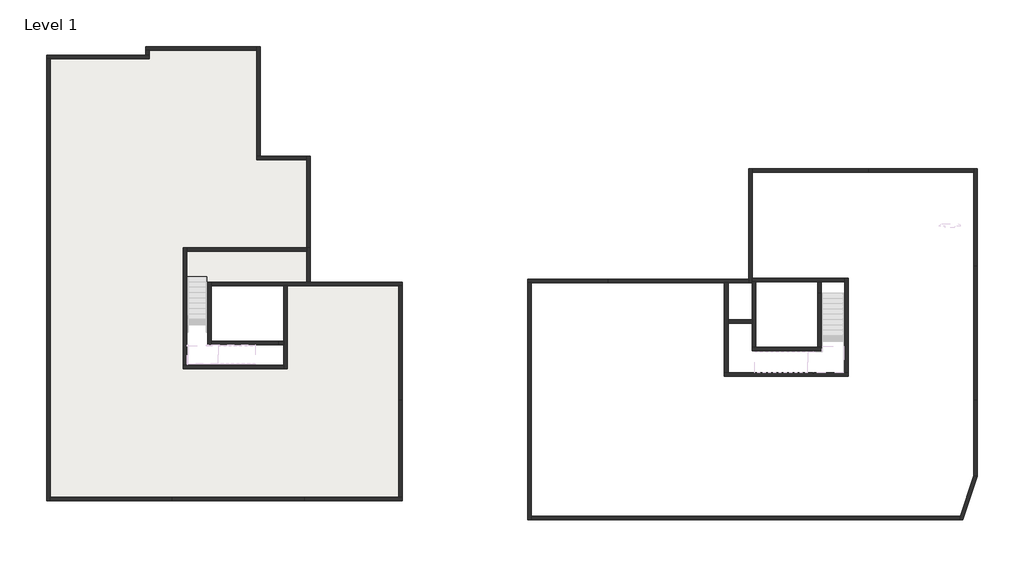
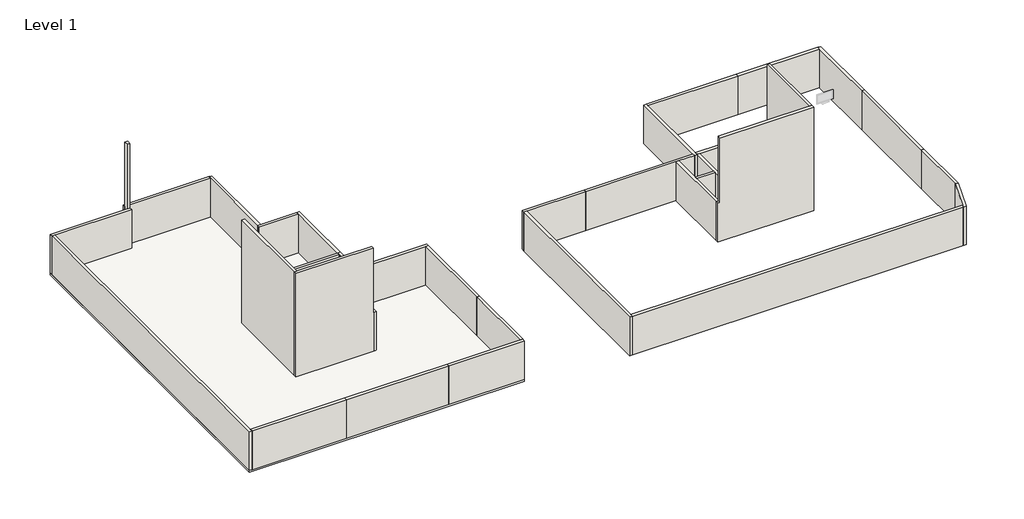
# One storey, part 1 of 2: 41 walls, 1 slab.
"""IFC4 building model written with IfcOpenShell, lengths in millimetres."""

from ifc_helpers import new_model, si_unit, frame, origin, origin_with_axes, place, context, project, spatial, polyline, outline, extrude, faceted_brep, element, save

model = new_model("IFC4")

# Units and contexts
model_context = context("Model", 3, world=origin())
ifc_project = project(units=[si_unit("LENGTHUNIT", "METRE", prefix="MILLI")], contexts=[model_context])

# Site, building, storey
site = spatial("IfcSite", under=ifc_project)
building = spatial("IfcBuilding", under=site)
storey = spatial("IfcBuildingStorey", under=building, Name="Level 1", Elevation=0.0)

# Slab
placement = place(None, origin())
element("IfcSlab", 1, ObjectType="Generic 150mm", at=placement, inside=storey, context=model_context, shape_type="SweptSolid", body=[
    extrude(outline(polyline([(-16680.1759629, 14256.1136739), (-16680.1759629, 14747.088776), (-10220.690523, 14747.088776), (-10220.690523, 8542.3434304), (-7387.4411293, 8542.3434304), (-7387.4411293, 1427.088776), (-2180.690523, 1427.088776), (-2180.690523, -10932.392509), (-22296.8569344, -10932.392509), (-22296.8569344, 14256.1136739), (-16680.1759629, 14256.1136739)]), holes=[polyline([(-8880.690523, -3253.8863261), (-8880.690523, 1227.088776), (-8880.690523, 1427.088776), (-14380.690523, 1427.088776), (-14380.690523, -3253.8863261), (-8880.690523, -3253.8863261)])]), frame((0.0, 0.0, -150.0), z_axis=(0.0, 0.0, 1.0), x_axis=(1.0, 0.0, 0.0)), (0.0, 0.0, 1.0), 150.0),
])

# Walls
element("IfcWall", 2, ObjectType="Generic - 200mm", at=placement, inside=storey, context=model_context, shape_type="SweptSolid", body=[
    extrude(outline(polyline([(30117.9969803, 7645.7271169), (24149.836337, 7645.7271169), (24149.836337, 7845.7271169), (30117.9969803, 7845.7271169), (30117.9969803, 7645.7271169)])), origin_with_axes(), (0.0, 0.0, 1.0), 3000.0),
])
element("IfcWall", 3, ObjectType="Generic - 200mm", at=placement, inside=storey, context=model_context, shape_type="Brep", body=[
    faceted_brep([(30117.9969803, 7845.7271169, 0.0), (30117.9969803, 7645.7271169, 0.0), (30117.9969803, 2319.475628, 0.0), (30117.9969803, 2319.475628, 3000.0), (30117.9969803, 7645.7271169, 3000.0), (30117.9969803, 7845.7271169, 3000.0), (30317.9969803, 7845.7271169, 0.0), (30317.9969803, 7845.7271169, 3000.0), (30317.9969803, 2319.475628, 3000.0), (30317.9969803, 2319.475628, 0.0), (30118.5156953, 2319.475628, 0.0), (30268.3425199, 2319.475628, 3000.0), (30118.5156953, 2319.475628, 3000.0)], [[[0, 1, 2, 3, 4, 5]], [[6, 7, 8, 9]], [[2, 1, 0, 6, 9, 10]], [[3, 2, 10, 9, 8, 11, 12]], [[5, 4, 3, 12, 11, 8, 7]], [[0, 5, 7, 6]]]),
])
element("IfcWall", 4, ObjectType="Generic - 200mm", at=placement, inside=storey, context=model_context, shape_type="Brep", body=[
    faceted_brep([(30118.5156953, 2319.475628, 0.0), (30118.5156953, -5240.0098119, 0.0), (30118.5156953, -5240.0098119, 3000.0), (30118.5156953, 2319.475628, 3000.0), (30318.5156953, 2319.475628, 0.0), (30318.5156953, 2319.475628, 3000.0), (30318.5156953, -5240.0098119, 3000.0), (30318.5156953, -5240.0098119, 0.0), (30317.9969803, 2319.475628, 0.0), (30119.0344102, -5240.0098119, 0.0), (30268.8612349, -5240.0098119, 3000.0), (30119.0344102, -5240.0098119, 3000.0), (30317.9969803, 2319.475628, 3000.0), (30268.8612349, 2319.475628, 3000.0)], [[[0, 1, 2, 3]], [[4, 5, 6, 7]], [[1, 0, 8, 4, 7, 9]], [[2, 1, 9, 7, 6, 10, 11]], [[3, 2, 11, 10, 6, 5, 12, 13]], [[0, 3, 13, 12, 5, 4, 8]]]),
])
element("IfcWall", 5, ObjectType="Generic - 200mm", at=placement, inside=storey, context=model_context, shape_type="Brep", body=[
    faceted_brep([(30119.0344102, -5240.0098119, 0.0), (30119.0344102, -9516.773704, 0.0), (30119.0344102, -9516.773704, 3000.0), (30119.0344102, -5240.0098119, 3000.0), (30319.0344102, -5240.0098119, 0.0), (30319.0344102, -5240.0098119, 3000.0), (30319.0344102, -9549.611954, 3000.0), (30319.0344102, -9549.611954, 0.0), (30318.5156953, -5240.0098119, 0.0), (30318.5156953, -5240.0098119, 3000.0), (30269.3799498, -5240.0098119, 3000.0)], [[[0, 1, 2, 3]], [[4, 5, 6, 7]], [[1, 0, 8, 4, 7]], [[3, 2, 6, 5, 9, 10]], [[0, 3, 10, 9, 5, 4, 8]], [[2, 1, 7, 6]]]),
])
element("IfcWall", 6, ObjectType="Generic - 200mm", at=placement, inside=storey, context=model_context, shape_type="Brep", body=[
    faceted_brep([(21499.4907974, -2250.0293367, 0.0), (21299.4907974, -2250.0293367, 0.0), (17780.2585618, -2250.0293367, 0.0), (17580.2585618, -2250.0293367, 0.0), (17580.2585618, -2250.0293367, 3000.0), (17780.2585618, -2250.0293367, 3000.0), (21299.4907974, -2250.0293367, 3000.0), (21499.4907974, -2250.0293367, 3000.0), (21499.4907974, -2450.0293367, 0.0), (21499.4907974, -2450.0293367, 3000.0), (17580.2585618, -2450.0293367, 3000.0), (17580.2585618, -2450.0293367, 0.0)], [[[0, 1, 2, 3, 4, 5, 6, 7]], [[8, 9, 10, 11]], [[3, 2, 1, 0, 8, 11]], [[7, 6, 5, 4, 10, 9]], [[4, 3, 11, 10]], [[0, 7, 9, 8]]]),
])
element("IfcWall", 7, ObjectType="Generic - 200mm", at=placement, inside=storey, context=model_context, shape_type="SweptSolid", body=[
    extrude(outline(polyline([(5093.3704674, -11810.4392945), (29344.9668625, -11810.4392945), (29277.4707506, -12010.4392945), (5093.3704674, -12010.4392945), (5093.3704674, -11810.4392945)])), origin_with_axes(), (0.0, 0.0, 1.0), 3000.0),
])
element("IfcWall", 8, ObjectType="Generic - 200mm", at=placement, inside=storey, context=model_context, shape_type="Brep", body=[
    faceted_brep([(30119.0344102, -9516.773704, 0.0), (29344.9668625, -11810.4392945, 0.0), (29277.4707506, -12010.4392945, 0.0), (29277.4707506, -12010.4392945, 3000.0), (29344.9668625, -11810.4392945, 3000.0), (30119.0344102, -9516.773704, 3000.0), (30319.0344102, -9549.611954, 0.0), (30319.0344102, -9549.611954, 3000.0), (29488.5530216, -12010.4392945, 3000.0), (29488.5530216, -12010.4392945, 0.0)], [[[0, 1, 2, 3, 4, 5]], [[6, 7, 8, 9]], [[2, 1, 0, 6, 9]], [[5, 4, 3, 8, 7]], [[0, 5, 7, 6]], [[3, 2, 9, 8]]]),
])
element("IfcWall", 9, ObjectType="Generic - 200mm", at=placement, inside=storey, context=model_context, shape_type="Brep", body=[
    faceted_brep([(4893.3704674, 1406.241677, 0.0), (4893.3704674, -12010.4392945, 0.0), (4893.3704674, -12010.4392945, 3000.0), (4893.3704674, 1406.241677, 3000.0), (5093.3704674, 1406.241677, 0.0), (5093.3704674, 1406.241677, 3000.0), (5093.3704674, -11810.4392945, 3000.0), (5093.3704674, -12010.4392945, 3000.0), (5093.3704674, -12010.4392945, 0.0), (5093.3704674, -11810.4392945, 0.0)], [[[0, 1, 2, 3]], [[4, 5, 6, 7, 8, 9]], [[1, 0, 4, 9, 8]], [[3, 2, 7, 6, 5]], [[2, 1, 8, 7]], [[0, 3, 5, 4]]]),
])
element("IfcWall", 10, ObjectType="Generic - 200mm", at=placement, inside=storey, context=model_context, shape_type="Brep", body=[
    faceted_brep([(21299.4907974, 799.475628, 0.0), (21299.4907974, -2250.0293367, 0.0), (21299.4907974, -2250.0293367, 3000.0), (21299.4907974, 799.475628, 3000.0), (21499.4907974, 799.475628, 0.0), (21499.4907974, 799.475628, 3000.0), (21499.4907974, -2250.0293367, 3000.0), (21499.4907974, -2250.0293367, 0.0), (21449.836337, 799.475628, 3000.0)], [[[0, 1, 2, 3]], [[4, 5, 6, 7]], [[1, 0, 4, 7]], [[3, 2, 6, 5, 8]], [[0, 3, 8, 5, 4]], [[2, 1, 7, 6]]]),
])
element("IfcWall", 11, ObjectType="Generic - 200mm", at=placement, inside=storey, context=model_context, shape_type="Brep", body=[
    faceted_brep([(17580.2585618, 1445.7271169, 0.0), (17580.2585618, -694.2728831, 0.0), (17580.2585618, -894.2728831, 0.0), (17580.2585618, -2250.0293367, 0.0), (17580.2585618, -2250.0293367, 3000.0), (17580.2585618, -894.2728831, 3000.0), (17580.2585618, -694.2728831, 3000.0), (17580.2585618, 1445.7271169, 3000.0), (17780.2585618, 1445.7271169, 0.0), (17780.2585618, 1445.7271169, 3000.0), (17780.2585618, -2250.0293367, 3000.0), (17780.2585618, -2250.0293367, 0.0)], [[[0, 1, 2, 3, 4, 5, 6, 7]], [[8, 9, 10, 11]], [[3, 2, 1, 0, 8, 11]], [[7, 6, 5, 4, 10, 9]], [[0, 7, 9, 8]], [[4, 3, 11, 10]]]),
])
element("IfcWall", 12, ObjectType="Generic - 200mm", at=placement, inside=storey, context=model_context, shape_type="Brep", body=[
    faceted_brep([(21499.4907974, 799.475628, 0.0), (21499.4907974, 1445.7271169, 0.0), (21499.4907974, 1445.7271169, 3000.0), (21499.4907974, 799.475628, 3000.0), (21299.4907974, 799.475628, 0.0), (21299.4907974, 799.475628, 3000.0), (21299.4907974, 1445.7271169, 3000.0), (21299.4907974, 1445.7271169, 0.0), (21449.836337, 799.475628, 3000.0)], [[[0, 1, 2, 3]], [[4, 5, 6, 7]], [[1, 0, 4, 7]], [[3, 2, 6, 5, 8]], [[0, 3, 8, 5, 4]], [[2, 1, 7, 6]]]),
])
element("IfcWall", 13, ObjectType="Generic - 200mm", at=placement, inside=storey, context=model_context, shape_type="SweptSolid", body=[
    extrude(outline(polyline([(24149.836337, 7645.7271169), (17578.5156953, 7645.7271169), (17578.5156953, 7845.7271169), (24149.836337, 7845.7271169), (24149.836337, 7645.7271169)])), origin_with_axes(), (0.0, 0.0, 1.0), 3000.0),
])
element("IfcWall", 14, ObjectType="Generic - 200mm", at=placement, inside=storey, context=model_context, shape_type="Brep", body=[
    faceted_brep([(16220.2585618, -3694.2728831, 0.0), (16220.2585618, -894.2728831, 0.0), (16220.2585618, -694.2728831, 0.0), (16220.2585618, 1405.7271169, 0.0), (16220.2585618, 1405.7271169, 3000.0), (16220.2585618, -694.2728831, 3000.0), (16220.2585618, -894.2728831, 3000.0), (16220.2585618, -3694.2728831, 3000.0), (16020.2585618, -3694.2728831, 0.0), (16020.2585618, -3694.2728831, 3000.0), (16020.2585618, 1405.7271169, 3000.0), (16020.2585618, 1405.7271169, 0.0), (16170.6041014, -3694.2728831, 3000.0)], [[[0, 1, 2, 3, 4, 5, 6, 7]], [[8, 9, 10, 11]], [[3, 2, 1, 0, 8, 11]], [[7, 6, 5, 4, 10, 9, 12]], [[4, 3, 11, 10]], [[0, 7, 12, 9, 8]]]),
])
element("IfcWall", 15, ObjectType="Generic - 200mm", at=placement, inside=storey, context=model_context, shape_type="SweptSolid", body=[
    extrude(outline(polyline([(17580.2585618, -894.2728831), (16220.2585618, -894.2728831), (16220.2585618, -694.2728831), (17580.2585618, -694.2728831), (17580.2585618, -894.2728831)])), origin_with_axes(), (0.0, 0.0, 1.0), 3000.0),
])
element("IfcWall", 16, ObjectType="Generic - 200mm", at=placement, inside=storey, context=model_context, shape_type="Brep", body=[
    faceted_brep([(17378.5156953, 7845.7271169, 0.0), (17378.5156953, 1605.7271169, 0.0), (17378.5156953, 1405.7271169, 0.0), (17378.5156953, 1405.7271169, 3000.0), (17378.5156953, 1605.7271169, 3000.0), (17378.5156953, 7845.7271169, 3000.0), (17578.5156953, 7845.7271169, 0.0), (17578.5156953, 7845.7271169, 3000.0), (17578.5156953, 7645.7271169, 3000.0), (17578.5156953, 1645.7271169, 3000.0), (17578.5156953, 1445.7271169, 3000.0), (17578.5156953, 1405.7271169, 3000.0), (17578.5156953, 1405.7271169, 0.0), (17578.5156953, 1445.7271169, 0.0), (17578.5156953, 1645.7271169, 0.0), (17578.5156953, 7645.7271169, 0.0)], [[[0, 1, 2, 3, 4, 5]], [[6, 7, 8, 9, 10, 11, 12, 13, 14, 15]], [[2, 1, 0, 6, 15, 14, 13, 12]], [[5, 4, 3, 11, 10, 9, 8, 7]], [[0, 5, 7, 6]], [[3, 2, 12, 11]]]),
])
element("IfcWall", 17, ObjectType="Generic - 200mm", at=placement, inside=storey, context=model_context, shape_type="Brep", body=[
    faceted_brep([(17378.5156953, 1605.7271169, 0.0), (9418.5156953, 1605.7271169, 0.0), (9418.5156953, 1605.7271169, 3000.0), (17378.5156953, 1605.7271169, 3000.0), (17378.5156953, 1405.7271169, 0.0), (17378.5156953, 1405.7271169, 3000.0), (16220.2585618, 1405.7271169, 3000.0), (16020.2585618, 1405.7271169, 3000.0), (9418.5156953, 1405.7271169, 3000.0), (9418.5156953, 1405.7271169, 0.0), (16020.2585618, 1405.7271169, 0.0), (16220.2585618, 1405.7271169, 0.0), (9418.5156953, 1406.241677, 0.0), (9418.5156953, 1406.241677, 3000.0)], [[[0, 1, 2, 3]], [[4, 5, 6, 7, 8, 9, 10, 11]], [[1, 0, 4, 11, 10, 9, 12]], [[2, 1, 12, 9, 8, 13]], [[3, 2, 13, 8, 7, 6, 5]], [[0, 3, 5, 4]]]),
])
element("IfcWall", 18, ObjectType="Generic - 200mm", at=placement, inside=storey, context=model_context, shape_type="Brep", body=[
    faceted_brep([(22820.2585618, 1645.7271169, 0.0), (17578.5156953, 1645.7271169, 0.0), (17578.5156953, 1645.7271169, 3000.0), (22820.2585618, 1645.7271169, 3000.0), (22820.2585618, 1445.7271169, 0.0), (22820.2585618, 1445.7271169, 3000.0), (21499.4907974, 1445.7271169, 3000.0), (21299.4907974, 1445.7271169, 3000.0), (17780.2585618, 1445.7271169, 3000.0), (17580.2585618, 1445.7271169, 3000.0), (17578.5156953, 1445.7271169, 3000.0), (17578.5156953, 1445.7271169, 0.0), (17580.2585618, 1445.7271169, 0.0), (17780.2585618, 1445.7271169, 0.0), (21299.4907974, 1445.7271169, 0.0), (21499.4907974, 1445.7271169, 0.0)], [[[0, 1, 2, 3]], [[4, 5, 6, 7, 8, 9, 10, 11, 12, 13, 14, 15]], [[1, 0, 4, 15, 14, 13, 12, 11]], [[3, 2, 10, 9, 8, 7, 6, 5]], [[2, 1, 11, 10]], [[0, 3, 5, 4]]]),
])
element("IfcWall", 19, ObjectType="Generic - 200mm", at=placement, inside=storey, context=model_context, shape_type="SweptSolid", body=[
    extrude(outline(polyline([(-2380.690523, -10732.392509), (-2380.690523, -5240.1378151), (-2180.690523, -5240.1378151), (-2180.690523, -10732.392509), (-2380.690523, -10732.392509)])), origin_with_axes(), (0.0, 0.0, 1.0), 3000.0),
])
element("IfcWall", 20, ObjectType="Generic - 200mm", at=placement, inside=storey, context=model_context, shape_type="Brep", body=[
    faceted_brep([(-2180.690523, -10732.392509, 0.0), (-2380.690523, -10732.392509, 0.0), (-7730.3449834, -10732.392509, 0.0), (-7730.3449834, -10732.392509, 3000.0), (-2380.690523, -10732.392509, 3000.0), (-2180.690523, -10732.392509, 3000.0), (-2180.690523, -10932.392509, 0.0), (-2180.690523, -10932.392509, 3000.0), (-7730.3449834, -10932.392509, 3000.0), (-7730.3449834, -10932.392509, 0.0), (-7730.3449834, -10732.911224, 0.0), (-7730.3449834, -10758.643998, 3000.0), (-7730.3449834, -10732.911224, 3000.0)], [[[0, 1, 2, 3, 4, 5]], [[6, 7, 8, 9]], [[2, 1, 0, 6, 9, 10]], [[3, 2, 10, 9, 8, 11, 12]], [[5, 4, 3, 12, 11, 8, 7]], [[0, 5, 7, 6]]]),
])
element("IfcWall", 21, ObjectType="Generic - 200mm", at=placement, inside=storey, context=model_context, shape_type="Brep", body=[
    faceted_brep([(-7730.3449834, -10732.911224, 0.0), (-15209.8304233, -10732.911224, 0.0), (-15209.8304233, -10732.911224, 3000.0), (-7730.3449834, -10732.911224, 3000.0), (-7730.3449834, -10932.911224, 0.0), (-7730.3449834, -10932.911224, 3000.0), (-15209.8304233, -10932.911224, 3000.0), (-15209.8304233, -10932.911224, 0.0), (-7730.3449834, -10932.392509, 0.0), (-15209.8304233, -10733.429939, 0.0), (-15209.8304233, -10759.1627129, 3000.0), (-15209.8304233, -10733.429939, 3000.0), (-7730.3449834, -10932.392509, 3000.0), (-7730.3449834, -10759.1627129, 3000.0)], [[[0, 1, 2, 3]], [[4, 5, 6, 7]], [[1, 0, 8, 4, 7, 9]], [[2, 1, 9, 7, 6, 10, 11]], [[3, 2, 11, 10, 6, 5, 12, 13]], [[0, 3, 13, 12, 5, 4, 8]]]),
])
element("IfcWall", 22, ObjectType="Generic - 200mm", at=placement, inside=storey, context=model_context, shape_type="Brep", body=[
    faceted_brep([(-15209.8304233, -10733.429939, 0.0), (-22096.8569344, -10733.429939, 0.0), (-22096.8569344, -10733.429939, 3000.0), (-15209.8304233, -10733.429939, 3000.0), (-15209.8304233, -10933.429939, 0.0), (-15209.8304233, -10933.429939, 3000.0), (-22096.8569344, -10933.429939, 3000.0), (-22096.8569344, -10933.429939, 0.0), (-15209.8304233, -10932.911224, 0.0), (-15209.8304233, -10932.911224, 3000.0), (-15209.8304233, -10759.6814279, 3000.0), (-15209.8304233, -10759.1627129, 3000.0)], [[[0, 1, 2, 3]], [[4, 5, 6, 7]], [[1, 0, 8, 4, 7]], [[3, 2, 6, 5, 9, 10, 11]], [[0, 3, 11, 10, 9, 5, 4, 8]], [[2, 1, 7, 6]]]),
])
element("IfcWall", 23, ObjectType="Generic - 200mm", at=placement, inside=storey, context=model_context, shape_type="Brep", body=[
    faceted_brep([(-12976.4469766, -2113.8863261, 0.0), (-12976.4469766, -1913.8863261, 0.0), (-12976.4469766, 1227.088776, 0.0), (-12976.4469766, 1427.088776, 0.0), (-12976.4469766, 1427.088776, 3000.0), (-12976.4469766, 1227.088776, 3000.0), (-12976.4469766, -1913.8863261, 3000.0), (-12976.4469766, -2113.8863261, 3000.0), (-13176.4469766, -2113.8863261, 0.0), (-13176.4469766, -2113.8863261, 3000.0), (-13176.4469766, 1427.088776, 3000.0), (-13176.4469766, 1427.088776, 0.0)], [[[0, 1, 2, 3, 4, 5, 6, 7]], [[8, 9, 10, 11]], [[3, 2, 1, 0, 8, 11]], [[7, 6, 5, 4, 10, 9]], [[4, 3, 11, 10]], [[0, 7, 9, 8]]]),
])
element("IfcWall", 24, ObjectType="Generic - 200mm", at=placement, inside=storey, context=model_context, shape_type="Brep", body=[
    faceted_brep([(-22096.8569344, -10933.429939, 0.0), (-22096.8569344, -10733.429939, 0.0), (-22096.8569344, 14056.1136739, 0.0), (-22096.8569344, 14056.1136739, 3000.0), (-22096.8569344, -10733.429939, 3000.0), (-22096.8569344, -10933.429939, 3000.0), (-22296.8569344, -10933.429939, 0.0), (-22296.8569344, -10933.429939, 3000.0), (-22296.8569344, 14056.1136739, 3000.0), (-22296.8569344, 14056.1136739, 0.0)], [[[0, 1, 2, 3, 4, 5]], [[6, 7, 8, 9]], [[2, 1, 0, 6, 9]], [[5, 4, 3, 8, 7]], [[0, 5, 7, 6]], [[3, 2, 9, 8]]]),
])
element("IfcWall", 25, ObjectType="Generic - 200mm", at=placement, inside=storey, context=model_context, shape_type="Brep", body=[
    faceted_brep([(-16480.1759629, 14256.1136739, 0.0), (-16680.1759629, 14256.1136739, 0.0), (-22296.8569344, 14256.1136739, 0.0), (-22296.8569344, 14256.1136739, 3000.0), (-16480.1759629, 14256.1136739, 3000.0), (-16480.1759629, 14056.1136739, 0.0), (-16480.1759629, 14056.1136739, 3000.0), (-22096.8569344, 14056.1136739, 3000.0), (-22296.8569344, 14056.1136739, 3000.0), (-22296.8569344, 14056.1136739, 0.0), (-22096.8569344, 14056.1136739, 0.0)], [[[0, 1, 2, 3, 4]], [[5, 6, 7, 8, 9, 10]], [[2, 1, 0, 5, 10, 9]], [[4, 3, 8, 7, 6]], [[3, 2, 9, 8]], [[0, 4, 6, 5]]]),
])
element("IfcWall", 26, ObjectType="Generic - 200mm", at=placement, inside=storey, context=model_context, shape_type="SweptSolid", body=[
    extrude(outline(polyline([(-12976.4469766, -1913.8863261), (-9200.690523, -1913.8863261), (-9200.690523, -2113.8863261), (-12976.4469766, -2113.8863261), (-12976.4469766, -1913.8863261)])), origin_with_axes(), (0.0, 0.0, 1.0), 3000.0),
])
element("IfcWall", 27, ObjectType="Generic - 200mm", at=placement, inside=storey, context=model_context, shape_type="SweptSolid", body=[
    extrude(outline(polyline([(-8880.690523, -2113.8863261), (-9200.690523, -2113.8863261), (-9200.690523, -1913.8863261), (-8880.690523, -1913.8863261), (-8880.690523, -2113.8863261)])), origin_with_axes(), (0.0, 0.0, 1.0), 3000.0),
])
element("IfcWall", 28, ObjectType="Generic - 200mm", at=placement, inside=storey, context=model_context, shape_type="SweptSolid", body=[
    extrude(outline(polyline([(-2380.690523, -5240.1378151), (-2380.690523, 1227.088776), (-2180.690523, 1227.088776), (-2180.690523, -5240.1378151), (-2380.690523, -5240.1378151)])), origin_with_axes(), (0.0, 0.0, 1.0), 3000.0),
])
element("IfcWall", 29, ObjectType="Generic - 200mm", at=placement, inside=storey, context=model_context, shape_type="SweptSolid", body=[
    extrude(outline(polyline([(-7580.690523, 3165.3459095), (-14380.690523, 3165.3459095), (-14380.690523, 3365.3459095), (-7580.690523, 3365.3459095), (-7580.690523, 3165.3459095)])), origin_with_axes(), (0.0, 0.0, 1.0), 3000.0),
])
element("IfcWall", 30, ObjectType="Generic - 200mm", at=placement, inside=storey, context=model_context, shape_type="Brep", body=[
    faceted_brep([(-2180.690523, 1427.088776, 0.0), (-7380.690523, 1427.088776, 0.0), (-7387.4411293, 1427.088776, 0.0), (-7580.690523, 1427.088776, 0.0), (-7587.4411293, 1427.088776, 0.0), (-12976.4469766, 1427.088776, 0.0), (-12976.4469766, 1427.088776, 3000.0), (-7587.4411293, 1427.088776, 3000.0), (-7580.690523, 1427.088776, 3000.0), (-7387.4411293, 1427.088776, 3000.0), (-7380.690523, 1427.088776, 3000.0), (-2180.690523, 1427.088776, 3000.0), (-2180.690523, 1227.088776, 0.0), (-2180.690523, 1227.088776, 3000.0), (-2380.690523, 1227.088776, 3000.0), (-8680.690523, 1227.088776, 3000.0), (-8880.690523, 1227.088776, 3000.0), (-12976.4469766, 1227.088776, 3000.0), (-12976.4469766, 1227.088776, 0.0), (-8880.690523, 1227.088776, 0.0), (-8680.690523, 1227.088776, 0.0), (-2380.690523, 1227.088776, 0.0)], [[[0, 1, 2, 3, 4, 5, 6, 7, 8, 9, 10, 11]], [[12, 13, 14, 15, 16, 17, 18, 19, 20, 21]], [[5, 4, 3, 2, 1, 0, 12, 21, 20, 19, 18]], [[11, 10, 9, 8, 7, 6, 17, 16, 15, 14, 13]], [[6, 5, 18, 17]], [[0, 11, 13, 12]]]),
])
element("IfcWall", 31, ObjectType="Generic - 200mm", at=placement, inside=storey, context=model_context, shape_type="Brep", body=[
    faceted_brep([(-7380.690523, 1427.088776, 0.0), (-7380.690523, 3367.088776, 0.0), (-7380.690523, 3367.088776, 3000.0), (-7380.690523, 1427.088776, 3000.0), (-7580.690523, 1427.088776, 0.0), (-7580.690523, 1427.088776, 3000.0), (-7580.690523, 3165.3459095, 3000.0), (-7580.690523, 3365.3459095, 3000.0), (-7580.690523, 3367.088776, 3000.0), (-7580.690523, 3367.088776, 0.0), (-7580.690523, 3365.3459095, 0.0), (-7580.690523, 3165.3459095, 0.0)], [[[0, 1, 2, 3]], [[4, 5, 6, 7, 8, 9, 10, 11]], [[1, 0, 4, 11, 10, 9]], [[2, 1, 9, 8]], [[3, 2, 8, 7, 6, 5]], [[0, 3, 5, 4]]]),
])
element("IfcWall", 32, ObjectType="Generic - 200mm", at=placement, inside=storey, context=model_context, shape_type="Brep", body=[
    faceted_brep([(-8680.690523, -3453.8863261, 0.0), (-8680.690523, 1227.088776, 0.0), (-8680.690523, 1227.088776, 3000.0), (-8680.690523, -3453.8863261, 3000.0), (-8880.690523, -3453.8863261, 0.0), (-8880.690523, -3453.8863261, 3000.0), (-8880.690523, -3253.8863261, 3000.0), (-8880.690523, -2113.8863261, 3000.0), (-8880.690523, -1913.8863261, 3000.0), (-8880.690523, 1227.088776, 3000.0), (-8880.690523, 1227.088776, 0.0), (-8880.690523, -1913.8863261, 0.0), (-8880.690523, -2113.8863261, 0.0), (-8880.690523, -3253.8863261, 0.0)], [[[0, 1, 2, 3]], [[4, 5, 6, 7, 8, 9, 10, 11, 12, 13]], [[1, 0, 4, 13, 12, 11, 10]], [[3, 2, 9, 8, 7, 6, 5]], [[2, 1, 10, 9]], [[0, 3, 5, 4]]]),
])
element("IfcWall", 33, ObjectType="Generic - 200mm", at=placement, inside=storey, context=model_context, shape_type="Brep", body=[
    faceted_brep([(9418.5156953, 1606.241677, 0.0), (4893.3704674, 1606.241677, 0.0), (4893.3704674, 1606.241677, 3000.0), (9418.5156953, 1606.241677, 3000.0), (9418.5156953, 1406.241677, 0.0), (9418.5156953, 1406.241677, 3000.0), (5093.3704674, 1406.241677, 3000.0), (4893.3704674, 1406.241677, 3000.0), (4893.3704674, 1406.241677, 0.0), (5093.3704674, 1406.241677, 0.0), (9418.5156953, 1605.7271169, 0.0), (9418.5156953, 1605.7271169, 3000.0)], [[[0, 1, 2, 3]], [[4, 5, 6, 7, 8, 9]], [[1, 0, 10, 4, 9, 8]], [[3, 2, 7, 6, 5, 11]], [[0, 3, 11, 5, 4, 10]], [[2, 1, 8, 7]]]),
])
element("IfcWall", 34, ObjectType="Generic - 200mm", at=placement, inside=storey, context=model_context, shape_type="Brep", body=[
    faceted_brep([(-10220.690523, 8542.3434304, 0.0), (-10220.690523, 14747.088776, 0.0), (-10220.690523, 14747.088776, 3000.0), (-10220.690523, 8542.3434304, 3000.0), (-10420.690523, 8542.3434304, 0.0), (-10420.690523, 8542.3434304, 3000.0), (-10420.690523, 14547.088776, 3000.0), (-10420.690523, 14747.088776, 3000.0), (-10420.690523, 14747.088776, 0.0), (-10420.690523, 14547.088776, 0.0)], [[[0, 1, 2, 3]], [[4, 5, 6, 7, 8, 9]], [[1, 0, 4, 9, 8]], [[3, 2, 7, 6, 5]], [[2, 1, 8, 7]], [[0, 3, 5, 4]]]),
])
element("IfcWall", 35, ObjectType="Generic - 200mm", at=placement, inside=storey, context=model_context, shape_type="Brep", body=[
    faceted_brep([(-10420.690523, 14747.088776, 0.0), (-16680.1759629, 14747.088776, 0.0), (-16680.1759629, 14747.088776, 3000.0), (-10420.690523, 14747.088776, 3000.0), (-10420.690523, 14547.088776, 0.0), (-10420.690523, 14547.088776, 3000.0), (-16680.1759629, 14547.088776, 3000.0), (-16680.1759629, 14547.088776, 0.0), (-16480.1759629, 14547.088776, 0.0)], [[[0, 1, 2, 3]], [[4, 5, 6, 7, 8]], [[1, 0, 4, 8, 7]], [[2, 1, 7, 6]], [[3, 2, 6, 5]], [[0, 3, 5, 4]]]),
])
element("IfcWall", 36, ObjectType="Generic - 200mm", at=placement, inside=storey, context=model_context, shape_type="Brep", body=[
    faceted_brep([(-8880.690523, -3253.8863261, 0.0), (-14380.690523, -3253.8863261, 0.0), (-14580.690523, -3253.8863261, 0.0), (-14580.690523, -3253.8863261, 8000.0), (-14380.690523, -3253.8863261, 8000.0), (-8930.3449834, -3253.8863261, 8000.0), (-8930.3449834, -3253.8863261, 3000.0), (-8880.690523, -3253.8863261, 3000.0), (-8880.690523, -3453.8863261, 0.0), (-8880.690523, -3453.8863261, 3000.0), (-8930.3449834, -3453.8863261, 3000.0), (-8930.3449834, -3453.8863261, 8000.0), (-14580.690523, -3453.8863261, 8000.0), (-14580.690523, -3453.8863261, 0.0), (-8930.3449834, -3280.1378151, 3000.0)], [[[0, 1, 2, 3, 4, 5, 6, 7]], [[8, 9, 10, 11, 12, 13]], [[2, 1, 0, 8, 13]], [[5, 4, 3, 12, 11]], [[6, 14, 10, 9, 7]], [[0, 7, 9, 8]], [[6, 5, 11, 10, 14]], [[3, 2, 13, 12]]]),
])
element("IfcWall", 37, ObjectType="Generic - 200mm", at=placement, inside=storey, context=model_context, shape_type="Brep", body=[
    faceted_brep([(-14380.690523, -3253.8863261, 0.0), (-14380.690523, 3165.3459095, 0.0), (-14380.690523, 3365.3459095, 0.0), (-14380.690523, 3365.3459095, 3000.0), (-14380.690523, 3365.3459095, 8000.0), (-14380.690523, -3253.8863261, 8000.0), (-14580.690523, -3253.8863261, 0.0), (-14580.690523, -3253.8863261, 8000.0), (-14580.690523, 3365.3459095, 8000.0), (-14580.690523, 3365.3459095, 0.0)], [[[0, 1, 2, 3, 4, 5]], [[6, 7, 8, 9]], [[2, 1, 0, 6, 9]], [[5, 4, 8, 7]], [[0, 5, 7, 6]], [[4, 3, 2, 9, 8]]]),
])
element("IfcWall", 38, ObjectType="Generic - 200mm", at=placement, inside=storey, context=model_context, shape_type="Brep", body=[
    faceted_brep([(-7387.4411293, 1427.088776, 0.0), (-7387.4411293, 8542.3434304, 0.0), (-7387.4411293, 8542.3434304, 3000.0), (-7387.4411293, 1427.088776, 3000.0), (-7587.4411293, 1427.088776, 0.0), (-7587.4411293, 1427.088776, 3000.0), (-7587.4411293, 8342.3434304, 3000.0), (-7587.4411293, 8542.3434304, 3000.0), (-7587.4411293, 8542.3434304, 0.0), (-7587.4411293, 8342.3434304, 0.0)], [[[0, 1, 2, 3]], [[4, 5, 6, 7, 8, 9]], [[1, 0, 4, 9, 8]], [[3, 2, 7, 6, 5]], [[2, 1, 8, 7]], [[0, 3, 5, 4]]]),
])
element("IfcWall", 39, ObjectType="Generic - 200mm", at=placement, inside=storey, context=model_context, shape_type="Brep", body=[
    faceted_brep([(-7587.4411293, 8542.3434304, 0.0), (-10220.690523, 8542.3434304, 0.0), (-10420.690523, 8542.3434304, 0.0), (-10427.4411293, 8542.3434304, 0.0), (-10427.4411293, 8542.3434304, 3000.0), (-10420.690523, 8542.3434304, 3000.0), (-10220.690523, 8542.3434304, 3000.0), (-7587.4411293, 8542.3434304, 3000.0), (-7587.4411293, 8342.3434304, 0.0), (-7587.4411293, 8342.3434304, 3000.0), (-10427.4411293, 8342.3434304, 3000.0), (-10427.4411293, 8342.3434304, 0.0)], [[[0, 1, 2, 3, 4, 5, 6, 7]], [[8, 9, 10, 11]], [[3, 2, 1, 0, 8, 11]], [[4, 3, 11, 10]], [[7, 6, 5, 4, 10, 9]], [[0, 7, 9, 8]]]),
])
element("IfcWall", 40, ObjectType="Generic - 200mm", at=placement, inside=storey, context=model_context, shape_type="Brep", body=[
    faceted_brep([(-16480.1759629, 14256.1136739, 0.0), (-16480.1759629, 14547.088776, 0.0), (-16480.1759629, 14547.088776, 8000.0), (-16480.1759629, 14256.1136739, 8000.0), (-16480.1759629, 14256.1136739, 3000.0), (-16680.1759629, 14256.1136739, 0.0), (-16680.1759629, 14256.1136739, 8000.0), (-16680.1759629, 14547.088776, 8000.0), (-16680.1759629, 14547.088776, 3000.0), (-16680.1759629, 14547.088776, 0.0)], [[[0, 1, 2, 3, 4]], [[5, 6, 7, 8, 9]], [[1, 0, 5, 9]], [[3, 2, 7, 6]], [[0, 4, 3, 6, 5]], [[2, 1, 9, 8, 7]]]),
])
element("IfcWall", 41, ObjectType="Generic - 200mm", at=placement, inside=storey, context=model_context, shape_type="Brep", body=[
    faceted_brep([(16020.2585618, -3894.2728831, 0.0), (23020.2585618, -3894.2728831, 0.0), (23020.2585618, -3894.2728831, 8000.0), (16170.6041014, -3894.2728831, 8000.0), (16170.6041014, -3894.2728831, 3000.0), (16020.2585618, -3894.2728831, 3000.0), (16020.2585618, -3694.2728831, 0.0), (16020.2585618, -3694.2728831, 3000.0), (16170.6041014, -3694.2728831, 3000.0), (16170.6041014, -3694.2728831, 8000.0), (22820.2585618, -3694.2728831, 8000.0), (23020.2585618, -3694.2728831, 8000.0), (23020.2585618, -3694.2728831, 0.0), (22820.2585618, -3694.2728831, 0.0), (16220.2585618, -3694.2728831, 0.0), (16170.6041014, -3740.0098119, 3000.0)], [[[0, 1, 2, 3, 4, 5]], [[6, 7, 8, 9, 10, 11, 12, 13, 14]], [[1, 0, 6, 14, 13, 12]], [[3, 2, 11, 10, 9]], [[4, 15, 8, 7, 5]], [[0, 5, 7, 6]], [[4, 3, 9, 8, 15]], [[2, 1, 12, 11]]]),
])
element("IfcWall", 42, ObjectType="Generic - 200mm", at=placement, inside=storey, context=model_context, shape_type="Brep", body=[
    faceted_brep([(23020.2585618, -3694.2728831, 0.0), (23020.2585618, 1645.7271169, 0.0), (23020.2585618, 1645.7271169, 8000.0), (23020.2585618, -3694.2728831, 8000.0), (22820.2585618, -3694.2728831, 0.0), (22820.2585618, -3694.2728831, 8000.0), (22820.2585618, 1645.7271169, 8000.0), (22820.2585618, 1645.7271169, 3000.0), (22820.2585618, 1645.7271169, 0.0), (22820.2585618, 1445.7271169, 0.0)], [[[0, 1, 2, 3]], [[4, 5, 6, 7, 8, 9]], [[1, 0, 4, 9, 8]], [[3, 2, 6, 5]], [[0, 3, 5, 4]], [[2, 1, 8, 7, 6]]]),
])

save(model, "model.ifc")

# Revit data of these elements
# Project information
#   Project Issue Date = "Issue Date"
#   Project Status = "Project Status"
#   Client Name = "Owner"
#   Project Address = "Enter address here"
#   Project Name = "Project Name"
#   Project Number = "0001"
# Type "Generic 150mm"
#   Function = 0
#   Layers, outside or top first: 15 cm no material (function 1)
# Type "Generic - 200mm"
#   Layers, outside or top first: 20 cm no material (function 1)
# Element 1 (IfcSlab, "Generic 150mm")
#   Height Offset From Level = 0 cm
#   Phase Created = New Construction
#   Materials on its faces: "Default Floor"
# Elements 2, 3, 4, 5, 6, 7, 8, 9, 10, 11, 12, 13, 14, 15, 16, 17, 18, 19, 20, 21, 22, 23, 24, 25, 26, 27, 28, 29, 30, 31, 32, 33, 34, 35, 38, 39 (IfcWall, "Generic - 200mm")
#   Top Offset = 0 cm
#   Base Offset = 0 cm
#   wall height = 300 cm
#   Phase Created = New Construction
#   Base Constraint = Level 1
#   Top Constraint = Level 2
#   Materials on its faces: "Default Wall"
# Elements 36, 37, 40, 41, 42 (IfcWall, "Generic - 200mm")
#   Top Offset = 0 cm
#   Base Offset = 0 cm
#   Unconnected Height = 800 cm
#   wall height = 800 cm
#   Phase Created = New Construction
#   Base Constraint = Level 1
#   Materials on its faces: "Default Wall"
# Materials
#   "Default Floor": class "Miscellaneous", colour RGB 127 127 127, transparency 0, Cost = 0
#   "Default Wall": class "Miscellaneous", colour RGB 128 128 128, transparency 0, Cost = 0
# Room, not placed, phase "New Construction", upper offset 0 cm, lower offset 0 cm
#   Number = "11"
#   Name = "Room"
# Room, not placed, phase "New Construction", upper offset 0 cm, lower offset 0 cm
#   Number = "12"
#   Name = "Room"
# Room, not placed, phase "New Construction", upper offset 0 cm, lower offset 0 cm
#   Number = "13"
#   Name = "Room"
# Room, not placed, phase "New Construction", upper offset 0 cm, lower offset 0 cm
#   Number = "14"
#   Name = "Room"
# Room, not placed, phase "New Construction", upper offset 0 cm, lower offset 0 cm
#   Number = "15"
#   Name = "Room"
# Room, not placed, phase "New Construction", upper offset 0 cm, lower offset 0 cm
#   Number = "16"
#   Name = "Room"
# Room, not placed, phase "New Construction", upper offset 0 cm, lower offset 0 cm
#   Number = "30"
#   Name = "Room"
# Room, not placed, phase "New Construction", upper offset 0 cm, lower offset 0 cm
#   Number = "31"
#   Name = "Room"
# Area, not placed, upper offset 0 cm, lower offset 0 cm
#   Number = "4"
#   Name = "Dere Parsel Toplam Alan"
# Room, not placed, phase "New Construction", upper offset 0 cm, lower offset 0 cm
#   Number = "106"
#   Name = "Room"
# Room, not placed, phase "New Construction", upper offset 0 cm, lower offset 0 cm
#   Number = "107"
#   Name = "Room"
# Room, not placed, phase "New Construction", upper offset 0 cm, lower offset 0 cm
#   Number = "109"
#   Name = "Room"
# Room, not placed, phase "New Construction", upper offset 0 cm, lower offset 0 cm
#   Number = "110"
#   Name = "7"
# Room, not placed, phase "New Construction", upper offset 0 cm, lower offset 0 cm
#   Number = "111"
#   Name = "8"
# Room, not placed, phase "New Construction", upper offset 0 cm, lower offset 0 cm
#   Number = "112"
#   Name = "9"
# Room, not placed, phase "New Construction", upper offset 0 cm, lower offset 0 cm
#   Number = "113"
#   Name = "1"
# Room, not placed, phase "New Construction", upper offset 0 cm, lower offset 0 cm
#   Number = "114"
#   Name = "5"
# Room, not placed, phase "New Construction", upper offset 0 cm, lower offset 0 cm
#   Number = "115"
#   Name = "2"
# Room, not placed, phase "New Construction", upper offset 0 cm, lower offset 0 cm
#   Number = "116"
#   Name = "4"
# Room, not placed, phase "New Construction", upper offset 0 cm, lower offset 0 cm
#   Number = "117"
#   Name = "3"
# Room, not placed, phase "New Construction", upper offset 0 cm, lower offset 0 cm
#   Number = "118"
#   Name = "6"
# Room, not placed, phase "New Construction", upper offset 0 cm, lower offset 0 cm
#   Number = "17"
#   Name = "Room"
# Room, not placed, phase "New Construction", upper offset 0 cm, lower offset 0 cm
#   Number = "119"
#   Name = "Room"
# Room, not placed, phase "New Construction", upper offset 0 cm, lower offset 0 cm
#   Number = "120"
#   Name = "Room"
# Room, not placed, phase "New Construction", upper offset 0 cm, lower offset 0 cm
#   Number = "77"
#   Name = "7"
# Room, not placed, phase "New Construction", upper offset 0 cm, lower offset 0 cm
#   Number = "78"
#   Name = "8"
# Room, not placed, phase "New Construction", upper offset 0 cm, lower offset 0 cm
#   Number = "79"
#   Name = "9"
# Room, not placed, phase "New Construction", upper offset 0 cm, lower offset 0 cm
#   Number = "80"
#   Name = "1"
# Room, not placed, phase "New Construction", upper offset 0 cm, lower offset 0 cm
#   Number = "81"
#   Name = "Room"
# Room, not placed, phase "New Construction", upper offset 0 cm, lower offset 0 cm
#   Number = "82"
#   Name = "Room"
# Room, not placed, phase "New Construction", upper offset 0 cm, lower offset 0 cm
#   Number = "83"
#   Name = "Room"
# Room, not placed, phase "New Construction", upper offset 0 cm, lower offset 0 cm
#   Number = "84"
#   Name = "5"
# Room, not placed, phase "New Construction", upper offset 0 cm, lower offset 0 cm
#   Number = "85"
#   Name = "Room"
# Room, not placed, phase "New Construction", upper offset 0 cm, lower offset 0 cm
#   Number = "137"
#   Name = "Room"
# Room, not placed, phase "New Construction", upper offset 0 cm, lower offset 0 cm
#   Number = "18"
#   Name = "Room"
# Room, not placed, phase "New Construction", upper offset 0 cm, lower offset 0 cm
#   Number = "86"
#   Name = "Room"
# Room, not placed, phase "New Construction", upper offset 0 cm, lower offset 0 cm
#   Number = "138"
#   Name = "Room"
# Room, not placed, phase "New Construction", upper offset 0 cm, lower offset 0 cm
#   Number = "139"
#   Name = "Room"
# Room, not placed, phase "New Construction", upper offset 0 cm, lower offset 0 cm
#   Number = "121"
#   Name = "Room"
# Room, not placed, phase "New Construction", upper offset 0 cm, lower offset 0 cm
#   Number = "122"
#   Name = "Room"
# Room, not placed, phase "New Construction", upper offset 0 cm, lower offset 0 cm
#   Number = ""
#   Name = "ASANSÖR"
# Room, not placed, phase "New Construction", upper offset 0 cm, lower offset 0 cm
#   Number = "49"
#   Name = "Room"
# Room, not placed, phase "New Construction", upper offset 0 cm, lower offset 0 cm
#   Number = "50"
#   Name = "Room"
# Room, not placed, phase "New Construction", upper offset 0 cm, lower offset 0 cm
#   Number = "51"
#   Name = "Room"
# Room, not placed, phase "New Construction", upper offset 0 cm, lower offset 0 cm
#   Number = "52"
#   Name = "Room"
# Room, not placed, phase "New Construction", upper offset 0 cm, lower offset 0 cm
#   Number = "53"
#   Name = "Room"
# Room, not placed, phase "New Construction", upper offset 0 cm, lower offset 0 cm
#   Number = "54"
#   Name = "Room"
# Room, not placed, phase "New Construction", upper offset 0 cm, lower offset 0 cm
#   Number = "55"
#   Name = "Room"
# Room, not placed, phase "New Construction", upper offset 0 cm, lower offset 0 cm
#   Number = "56"
#   Name = "Room"
# Room, not placed, phase "New Construction", upper offset 0 cm, lower offset 0 cm
#   Number = ""
#   Name = "Çamaşır- Kombi"
# Room, not placed, phase "New Construction", upper offset 0 cm, lower offset 0 cm
#   Number = "32"
#   Name = "Room"
# Room, not placed, phase "New Construction", upper offset 0 cm, lower offset 0 cm
#   Number = "33"
#   Name = "Room"
# Room, not placed, phase "New Construction", upper offset 0 cm, lower offset 0 cm
#   Number = "123"
#   Name = "Room"
# Room, not placed, phase "New Construction", upper offset 0 cm, lower offset 0 cm
#   Number = "87"
#   Name = "2"
# Room, not placed, phase "New Construction", upper offset 0 cm, lower offset 0 cm
#   Number = "88"
#   Name = "4"
# Room, not placed, phase "New Construction", upper offset 0 cm, lower offset 0 cm
#   Number = "57"
#   Name = "Room"
# Room, not placed, phase "New Construction", upper offset 0 cm, lower offset 0 cm
#   Number = ""
#   Name = "Room"
# Room, not placed, phase "New Construction", upper offset 0 cm, lower offset 0 cm
#   Number = "59"
#   Name = "Room"
# Room, not placed, phase "New Construction", upper offset 0 cm, lower offset 0 cm
#   Number = "60"
#   Name = "Room"
# Room, not placed, phase "New Construction", upper offset 0 cm, lower offset 0 cm
#   Number = "61"
#   Name = "Room"
# Room, not placed, phase "New Construction", upper offset 0 cm, lower offset 0 cm
#   Number = "62"
#   Name = "Room"
# Room, not placed, phase "New Construction", upper offset 0 cm, lower offset 0 cm
#   Number = "63"
#   Name = "Room"
# Area, not placed, upper offset 0 cm, lower offset 0 cm
#   Number = "5"
#   Name = "Dere Parsel Toplam Alan"
# Room, not placed, phase "New Construction", upper offset 0 cm, lower offset 0 cm
#   Number = "67"
#   Name = "Room"
# Room, not placed, phase "New Construction", upper offset 0 cm, lower offset 0 cm
#   Number = "68"
#   Name = "Room"
# Room, not placed, phase "New Construction", upper offset 0 cm, lower offset 0 cm
#   Number = "90"
#   Name = "3"
# Area, not placed, upper offset 0 cm, lower offset 0 cm
#   Number = "6"
#   Name = "Area"
# Room, not placed, phase "New Construction", upper offset 0 cm, lower offset 0 cm
#   Number = "93"
#   Name = "6"
# Room, not placed, phase "New Construction", upper offset 0 cm, lower offset 0 cm
#   Number = "5"
#   Name = "Room"
# Room, not placed, phase "New Construction", upper offset 0 cm, lower offset 0 cm
#   Number = "6"
#   Name = "Room"
# Room, not placed, phase "New Construction", upper offset 0 cm, lower offset 0 cm
#   Number = "124"
#   Name = "Room"
# Room, not placed, phase "New Construction", upper offset 0 cm, lower offset 0 cm
#   Number = "34"
#   Name = "Room"
# Room, not placed, phase "New Construction", upper offset 0 cm, lower offset 0 cm
#   Number = "35"
#   Name = "Room"
# Room, not placed, phase "New Construction", upper offset 0 cm, lower offset 0 cm
#   Number = "9"
#   Name = "Room"
# Room, not placed, phase "New Construction", upper offset 0 cm, lower offset 0 cm
#   Number = "10"
#   Name = "Room"
# Room, not placed, phase "New Construction", upper offset 0 cm, lower offset 0 cm
#   Number = "125"
#   Name = "Room"
# Room, not placed, phase "New Construction", upper offset 0 cm, lower offset 0 cm
#   Number = "126"
#   Name = "Room"
# Room, not placed, phase "New Construction", upper offset 0 cm, lower offset 0 cm
#   Number = "127"
#   Name = "Room"
# Room, not placed, phase "New Construction", upper offset 0 cm, lower offset 0 cm
#   Number = "128"
#   Name = "Room"
# Room, not placed, phase "New Construction", upper offset 0 cm, lower offset 0 cm
#   Number = "129"
#   Name = "Room"
# Room, not placed, phase "New Construction", upper offset 0 cm, lower offset 0 cm
#   Number = "91"
#   Name = "Room"
# Room, not placed, phase "New Construction", upper offset 0 cm, lower offset 0 cm
#   Number = "130"
#   Name = "Room"
# Room, not placed, phase "New Construction", upper offset 0 cm, lower offset 0 cm
#   Number = "131"
#   Name = "Room"
# Room, not placed, phase "New Construction", upper offset 0 cm, lower offset 0 cm
#   Number = "132"
#   Name = "Room"
# Room, not placed, phase "New Construction", upper offset 0 cm, lower offset 0 cm
#   Number = "133"
#   Name = "Room"
# Room, not placed, phase "New Construction", upper offset 0 cm, lower offset 0 cm
#   Number = ""
#   Name = ""
# Room, not placed, phase "New Construction", upper offset 0 cm, lower offset 0 cm
#   Number = "70"
#   Name = "Room"
# Room, not placed, phase "New Construction", upper offset 0 cm, lower offset 0 cm
#   Number = "71"
#   Name = "Room"
# Room, not placed, phase "New Construction", upper offset 0 cm, lower offset 0 cm
#   Number = "92"
#   Name = "Room"
# Room, not placed, phase "New Construction", upper offset 0 cm, lower offset 0 cm
#   Number = ""
#   Name = ""
# Room, not placed, phase "New Construction", upper offset 0 cm, lower offset 0 cm
#   Number = ""
#   Name = ""
# Room, not placed, phase "New Construction", upper offset 0 cm, lower offset 0 cm
#   Number = "37"
#   Name = "Room"
# Room, not placed, phase "New Construction", upper offset 0 cm, lower offset 0 cm
#   Number = ""
#   Name = "Banyo"
# Room, not placed, phase "New Construction", upper offset 0 cm, lower offset 0 cm
#   Number = ""
#   Name = ""
# Room, not placed, phase "New Construction", upper offset 0 cm, lower offset 0 cm
#   Number = ""
#   Name = "Yatak Odası"
# Room, not placed, phase "New Construction", upper offset 0 cm, lower offset 0 cm
#   Number = "39"
#   Name = "Room"
# Room, not placed, phase "New Construction", upper offset 0 cm, lower offset 0 cm
#   Number = ""
#   Name = "Salon-Mutfak"
# Area, not placed, upper offset 0 cm, lower offset 0 cm
#   Number = "9"
#   Name = "Area"
# Room, not placed, phase "New Construction", upper offset 0 cm, lower offset 0 cm
#   Number = "134"
#   Name = "Room"
# Room, not placed, phase "New Construction", upper offset 0 cm, lower offset 0 cm
#   Number = "135"
#   Name = "Room"
# Room, not placed, phase "New Construction", upper offset 0 cm, lower offset 0 cm
#   Number = "40"
#   Name = "Room"
# Room, not placed, phase "New Construction", upper offset 0 cm, lower offset 0 cm
#   Number = "41"
#   Name = "Room"
# Area, not placed, upper offset 0 cm, lower offset 0 cm
#   Number = "8"
#   Name = "Dere Parsel Toplam Alan"
# Room, not placed, phase "New Construction", upper offset 0 cm, lower offset 0 cm
#   Number = "108"
#   Name = "ASANSÖR"
# Room, not placed, phase "New Construction", upper offset 0 cm, lower offset 0 cm
#   Number = "89"
#   Name = "Room"
# Room, not placed, phase "New Construction", upper offset 0 cm, lower offset 0 cm
#   Number = "19"
#   Name = "Room"
# Room, not placed, phase "New Construction", upper offset 0 cm, lower offset 0 cm
#   Number = ""
#   Name = ""
# Room, not placed, phase "New Construction", upper offset 0 cm, lower offset 0 cm
#   Number = "21"
#   Name = "Room"
# Room, not placed, phase "New Construction", upper offset 0 cm, lower offset 0 cm
#   Number = "22"
#   Name = "Room"
# Room, not placed, phase "New Construction", upper offset 0 cm, lower offset 0 cm
#   Number = "23"
#   Name = "Room"
# Room, not placed, phase "New Construction", upper offset 0 cm, lower offset 0 cm
#   Number = "24"
#   Name = "Room"
# Room, not placed, phase "New Construction", upper offset 0 cm, lower offset 0 cm
#   Number = "25"
#   Name = "Room"
# Room, not placed, phase "New Construction", upper offset 0 cm, lower offset 0 cm
#   Number = "64"
#   Name = "Room"
# Room, not placed, phase "New Construction", upper offset 0 cm, lower offset 0 cm
#   Number = "65"
#   Name = "Room"
# Room, not placed, phase "New Construction", upper offset 0 cm, lower offset 0 cm
#   Number = "66"
#   Name = "Room"
# Room, not placed, phase "New Construction", upper offset 0 cm, lower offset 0 cm
#   Number = ""
#   Name = ""
# Room, not placed, phase "New Construction", upper offset 0 cm, lower offset 0 cm
#   Number = "27"
#   Name = "Room"
# Room, not placed, phase "New Construction", upper offset 0 cm, lower offset 0 cm
#   Number = "42"
#   Name = "Room"
# Area, not placed, upper offset 0 cm, lower offset 0 cm
#   Number = "2"
#   Name = "Area"
# Room, not placed, phase "New Construction", upper offset 0 cm, lower offset 0 cm
#   Number = "43"
#   Name = "Room"
# Room, not placed, phase "New Construction", upper offset 0 cm, lower offset 0 cm
#   Number = ""
#   Name = ""
# Room, not placed, phase "New Construction", upper offset 0 cm, lower offset 0 cm
#   Number = "94"
#   Name = "Room"
# Room, not placed, phase "New Construction", upper offset 0 cm, lower offset 0 cm
#   Number = ""
#   Name = ""
# Room, not placed, phase "New Construction", upper offset 0 cm, lower offset 0 cm
#   Number = "136"
#   Name = "Room"
# Room, not placed, phase "New Construction", upper offset 0 cm, lower offset 0 cm
#   Number = "1"
#   Name = "Room"
# Area, not placed, upper offset 0 cm, lower offset 0 cm
#   Number = "3"
#   Name = "Area"
# Room, not placed, phase "New Construction", upper offset 0 cm, lower offset 0 cm
#   Number = "7"
#   Name = "Room"
# Room, not placed, phase "New Construction", upper offset 0 cm, lower offset 0 cm
#   Number = "8"
#   Name = "Room"
# Room, not placed, phase "New Construction", upper offset 0 cm, lower offset 0 cm
#   Number = "2"
#   Name = "Room"
# Room, not placed, phase "New Construction", upper offset 0 cm, lower offset 0 cm
#   Number = "46"
#   Name = "Room"
# Room, not placed, phase "New Construction", upper offset 0 cm, lower offset 0 cm
#   Number = "3"
#   Name = "Room"
# Room, not placed, phase "New Construction", upper offset 0 cm, lower offset 0 cm
#   Number = ""
#   Name = ""
# Room, not placed, phase "New Construction", upper offset 0 cm, lower offset 0 cm
#   Number = "4"
#   Name = "Room"
# Area, not placed, upper offset 0 cm, lower offset 0 cm
#   Number = "1"
#   Name = "Area"
# Room, not placed, phase "New Construction", upper offset 0 cm, lower offset 0 cm
#   Number = ""
#   Name = ""
# Room, not placed, phase "New Construction", upper offset 0 cm, lower offset 0 cm
#   Number = "29"
#   Name = "Room"
# Area, not placed, upper offset 0 cm, lower offset 0 cm
#   Number = "7"
#   Name = "Dere Parsel Toplam Alan"
# Room, not placed, phase "New Construction", upper offset 0 cm, lower offset 0 cm
#   Number = "95"
#   Name = "ASANSÖR"
# Room, not placed, phase "New Construction", upper offset 0 cm, lower offset 0 cm
#   Number = "96"
#   Name = "Room"
# Room, not placed, phase "New Construction", upper offset 0 cm, lower offset 0 cm
#   Number = "97"
#   Name = "7"
# Room, not placed, phase "New Construction", upper offset 0 cm, lower offset 0 cm
#   Number = "98"
#   Name = "8"
# Room, not placed, phase "New Construction", upper offset 0 cm, lower offset 0 cm
#   Number = "99"
#   Name = "9"
# Room, not placed, phase "New Construction", upper offset 0 cm, lower offset 0 cm
#   Number = "100"
#   Name = "1"
# Room, not placed, phase "New Construction", upper offset 0 cm, lower offset 0 cm
#   Number = "101"
#   Name = "5"
# Room, not placed, phase "New Construction", upper offset 0 cm, lower offset 0 cm
#   Number = "102"
#   Name = "2"
# Room, not placed, phase "New Construction", upper offset 0 cm, lower offset 0 cm
#   Number = "103"
#   Name = "4"
# Room, not placed, phase "New Construction", upper offset 0 cm, lower offset 0 cm
#   Number = "104"
#   Name = "3"
# Room, not placed, phase "New Construction", upper offset 0 cm, lower offset 0 cm
#   Number = "105"
#   Name = "6"
